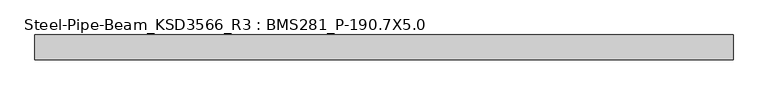
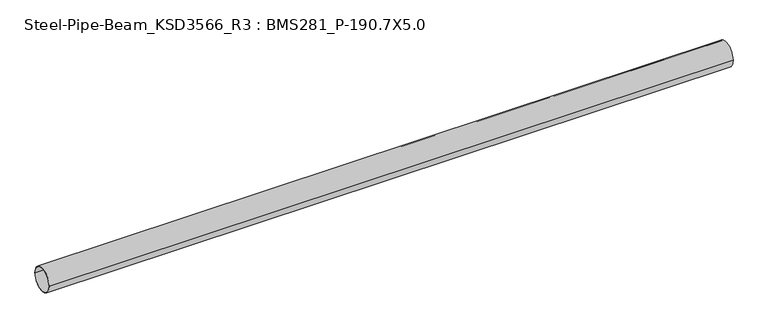
"""IFC4 building model written with IfcOpenShell, lengths in millimetres: member geometry, Steel-Pipe-Beam_KSD3566_R3 : BMS281_P-190.7X5.0."""

from ifc_helpers import new_model, si_unit, point, frame, origin, origin_2d, place, context, project, spatial, circle_curve, trimmed, segment, composite_curve, outline, extrude, source, transform, mapped, element, save


def steel_pipe_beam_ksd3566_r3_bms281_p_190_7x5_0_d445f5b3(model_context):
    return source(origin(), model_context, "Body", "SweptSolid", [
        extrude(outline(composite_curve([segment(trimmed(circle_curve(origin_2d(), 95.35), [point((-95.35, 0.0))], [point((95.35, 0.0))], False, "CARTESIAN"), True, "CONTINUOUS"), segment(trimmed(circle_curve(origin_2d(), 95.35), [point((95.35, 0.0))], [point((-95.35, 0.0))], False, "CARTESIAN"), True, "CONTINUOUS")], self_intersect=False), holes=[composite_curve([segment(trimmed(circle_curve(origin_2d(), 90.35), [point((90.35, 0.0))], [point((-90.35, 0.0))], True, "CARTESIAN"), True, "CONTINUOUS"), segment(trimmed(circle_curve(origin_2d(), 90.35), [point((-90.35, 0.0))], [point((90.35, 0.0))], True, "CARTESIAN"), True, "CONTINUOUS")], self_intersect=False)]), frame((-2743.0186842, 0.0, 0.0), z_axis=(1.0, 0.0, 0.0), x_axis=(0.0, 1.0, 0.0)), (0.0, 0.0, 1.0), 5331.5201088),
    ])


if __name__ == "__main__":
    model = new_model("IFC4")
    model_context = context("Model", 3, world=origin())
    ifc_project = project(units=[si_unit("LENGTHUNIT", "METRE", prefix="MILLI")], contexts=[model_context])
    site = spatial("IfcSite", under=ifc_project)
    building = spatial("IfcBuilding", under=site)
    placement = place(None, origin())
    steel_pipe_beam_ksd3566_r3_bms281_p_190_7x5_0_shape = steel_pipe_beam_ksd3566_r3_bms281_p_190_7x5_0_d445f5b3(model_context)
    element("IfcMember", 1, ObjectType="Steel-Pipe-Beam_KSD3566_R3 : BMS281_P-190.7X5.0", at=placement, inside=building, context=model_context, shape_type="MappedRepresentation", body=[
        mapped(steel_pipe_beam_ksd3566_r3_bms281_p_190_7x5_0_shape, transform((0.0, 0.0, 0.0), x_axis=(1.0, 0.0, 0.0), y_axis=(0.0, 1.0, 0.0), z_axis=(0.0, 0.0, 1.0))),
    ])
    save(model, "model.ifc")

# Revit data of these elements
# Type "Steel-Pipe-Beam_KSD3566_R3 : BMS281_P-190.7X5.0"
#   Keynote = "P-190.7X5.0"
#   SteelWeight = "Light"
#   t = 0.0050 m
#   Surface Area = 0.599102 m²/m
#   Section Area = 29.1697 cm²
#   Mass per Unit Length = 22.8982 kg/m
#   Length [instance default] = 1.5000 m
#   D = 0.1907 m
#   hec_material4 [instance default] = none
#   hec_material3 [instance default] = none
#   hec_material2 [instance default] = none
#   hec_material1 [instance default] = none
#   Structural Material [instance default] = Steel, 45-345
#   Assembly Code = ""
# Element 1 (IfcMember, "Steel-Pipe-Beam_KSD3566_R3 : BMS281_P-190.7X5.0")
#   Structural Material = none
# Materials
#   "Steel, 45-345": class "Metal", colour RGB 189 187 185, transparency 0, Description = "Steel 345 MPa", Cost = 0
